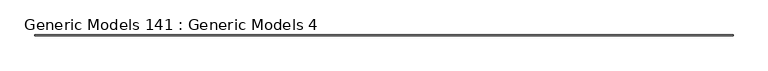
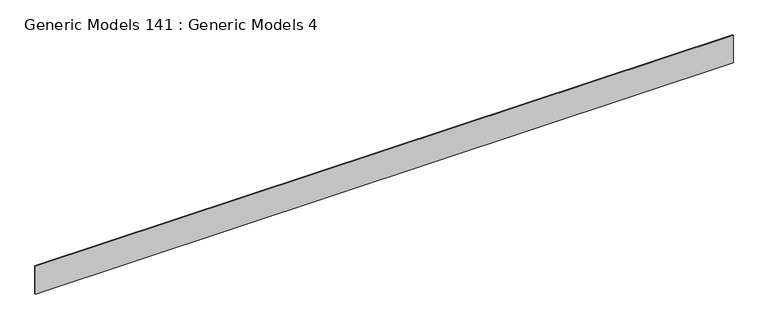
"""IFC4 building model written with IfcOpenShell, lengths in millimetres: proxy geometry, Generic Models 141 : Generic Models 4."""

from ifc_helpers import new_model, si_unit, frame, origin, place, context, project, spatial, polyline, outline, extrude, source, transform, mapped, element, save


def generic_models_141_generic_models_4_645eafa7(model_context):
    return source(origin(), model_context, "Body", "SweptSolid", [
        extrude(outline(polyline([(-2152.1733045, 51452.647716), (-2152.1733045, 51433.597716), (-20795.7733045, 51433.597716), (-20795.7733045, 51452.647716), (-2152.1733045, 51452.647716)])), frame((0.0, 0.0, 126384.0358061), z_axis=(0.0, 0.0, 1.0), x_axis=(1.0, 0.0, 0.0)), (0.0, 0.0, 1.0), 780.3940166),
    ])


if __name__ == "__main__":
    model = new_model("IFC4")
    model_context = context("Model", 3, world=origin())
    ifc_project = project(units=[si_unit("LENGTHUNIT", "METRE", prefix="MILLI")], contexts=[model_context])
    site = spatial("IfcSite", under=ifc_project)
    building = spatial("IfcBuilding", under=site)
    placement = place(None, origin())
    generic_models_141_generic_models_4_shape = generic_models_141_generic_models_4_645eafa7(model_context)
    element("IfcBuildingElementProxy", 1, Name="Generic Models 141 : Generic Models 4", ObjectType="Generic Models 141 : Generic Models 4", at=placement, inside=building, context=model_context, shape_type="MappedRepresentation", body=[
        mapped(generic_models_141_generic_models_4_shape, transform((0.0, 0.0, 0.0), x_axis=(1.0, 0.0, 0.0), y_axis=(0.0, 1.0, 0.0), z_axis=(0.0, 0.0, 1.0))),
    ])
    save(model, "model.ifc")

# Revit data of these elements
# Element 1 (IfcBuildingElementProxy, "Generic Models 141 : Generic Models 4")
#   Materials on its faces: "_CDX PLYWOOD - SEE STRUCT DWGs"
# Materials
#   "_CDX PLYWOOD - SEE STRUCT DWGs": class "Generic", colour RGB 98 75 74, transparency 0, Cost = 0
